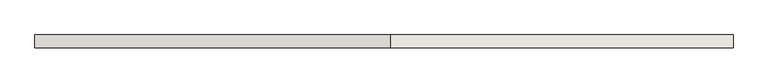
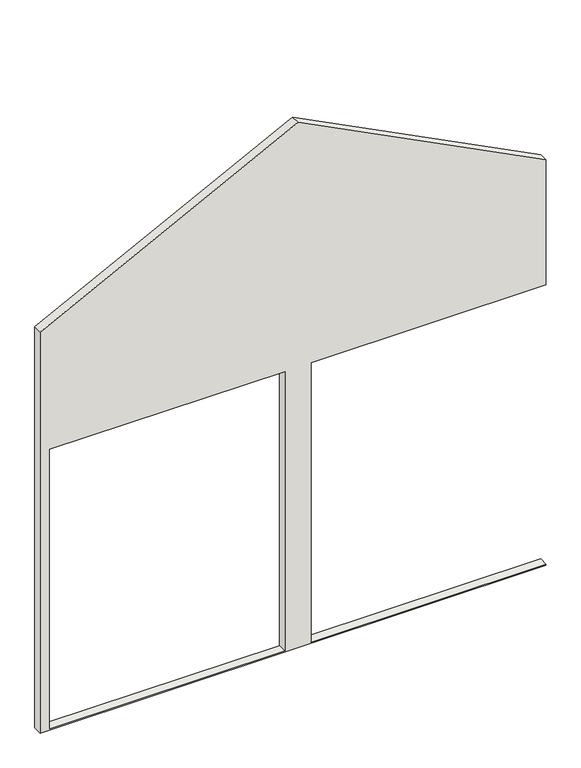
"""IFC4 building model written with IfcOpenShell, lengths in millimetres: wall geometry, 0_3d."""

from ifc_helpers import new_model, si_unit, frame, origin, place, context, project, spatial, polyline, outline, extrude, source, transform, mapped, element, save


def wall_3b7ee32a(model_context):
    return source(origin(), model_context, "Body", "SweptSolid", [
        extrude(outline(polyline([(10.0, 3875.0), (10.0, 2075.0), (2270.0, 2075.0), (2270.0, 3875.0), (3283.5797924, 3875.0), (4251.6781465, 1975.0), (3245.3653837, 0.0), (0.0, 0.0), (0.0, 3875.0), (10.0, 3875.0)]), holes=[polyline([(2270.0, 1875.0), (10.0, 1875.0), (10.0, 75.0), (2270.0, 75.0), (2270.0, 1875.0)])]), frame((0.0, 0.0, 0.0), z_axis=(0.0, 1.0, 0.0), x_axis=(0.0, 0.0, 1.0)), (0.0, 0.0, 1.0), 70.0),
    ])


if __name__ == "__main__":
    model = new_model("IFC4")
    model_context = context("Model", 3, world=origin())
    ifc_project = project(units=[si_unit("LENGTHUNIT", "METRE", prefix="MILLI")], contexts=[model_context])
    site = spatial("IfcSite", under=ifc_project)
    building = spatial("IfcBuilding", under=site)
    placement = place(None, origin())
    wall_shape = wall_3b7ee32a(model_context)
    element("IfcWall", 1, ObjectType="0_3d", at=placement, inside=building, context=model_context, shape_type="MappedRepresentation", body=[
        mapped(wall_shape, transform((0.0, 0.0, 0.0), x_axis=(1.0, 0.0, 0.0), y_axis=(0.0, 1.0, 0.0), z_axis=(0.0, 0.0, 1.0))),
    ])
    save(model, "model.ifc")

# Revit data of these elements
# Element 1 (IfcWall, "0_3d")
#   Materials on its faces: "Glass_Simple"
# Materials
#   "Glass_Simple": class "Unassigned", colour RGB 255 255 255, transparency 0.9
